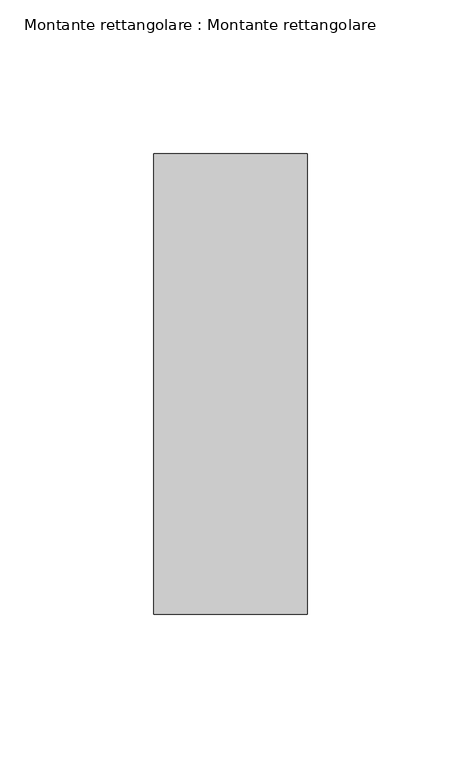
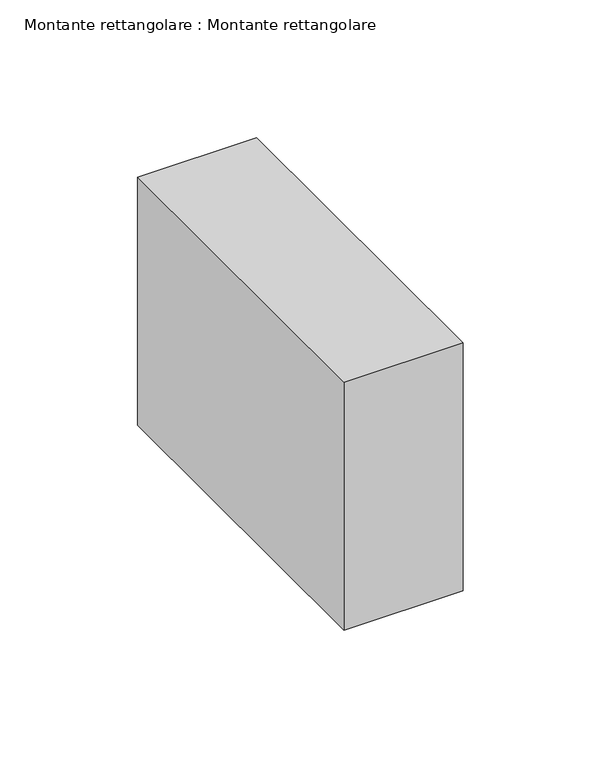
"""IFC4 building model written with IfcOpenShell, lengths in millimetres: member geometry, Montante rettangolare : Montante rettangolare."""

from ifc_helpers import new_model, si_unit, frame, origin, place, context, project, spatial, polyline, outline, extrude, source, transform, mapped, element, save


def montante_rettangolare_montante_rettangolare_244bd407(model_context):
    return source(origin(), model_context, "Body", "SweptSolid", [
        extrude(outline(polyline([(0.0, 75.0), (0.0, -75.0), (-50.0, -75.0), (-50.0, 75.0), (0.0, 75.0)])), frame((0.0, 0.0, -110.0), z_axis=(0.0, 0.0, 1.0), x_axis=(1.0, 0.0, 0.0)), (0.0, 0.0, 1.0), 110.0),
    ])


if __name__ == "__main__":
    model = new_model("IFC4")
    model_context = context("Model", 3, world=origin())
    ifc_project = project(units=[si_unit("LENGTHUNIT", "METRE", prefix="MILLI")], contexts=[model_context])
    site = spatial("IfcSite", under=ifc_project)
    building = spatial("IfcBuilding", under=site)
    placement = place(None, origin())
    montante_rettangolare_montante_rettangolare_shape = montante_rettangolare_montante_rettangolare_244bd407(model_context)
    element("IfcMember", 1, ObjectType="Montante rettangolare : Montante rettangolare", at=placement, inside=building, context=model_context, shape_type="MappedRepresentation", body=[
        mapped(montante_rettangolare_montante_rettangolare_shape, transform((0.0, 0.0, 0.0), x_axis=(1.0, 0.0, 0.0), y_axis=(0.0, 1.0, 0.0), z_axis=(0.0, 0.0, 1.0))),
    ])
    save(model, "model.ifc")

# Revit data of these elements
# Type "Montante rettangolare : Montante rettangolare"
#   built-in parameter 1007304 = 0.492126 (stored number, unit not read)
#   built-in parameter 1007301 = 0.082021 (stored number, unit not read)
#   built-in parameter 1007300 = 0.082021 (stored number, unit not read)
# Element 1 (IfcMember, "Montante rettangolare : Montante rettangolare")
#   Materials on its faces: "Acciaio"
# Materials
#   "Acciaio": class "Metallo", colour RGB 247 247 247, transparency 0, Description = "Acciaio, finitura zigrinata", Cost = 0
